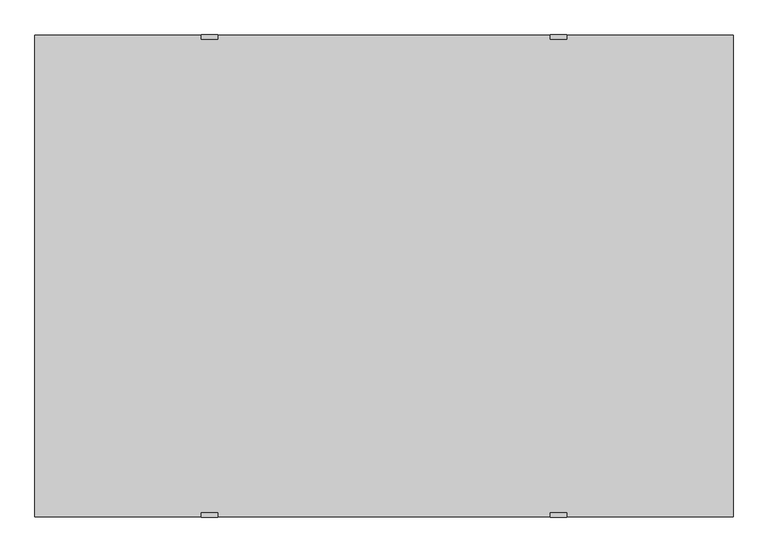
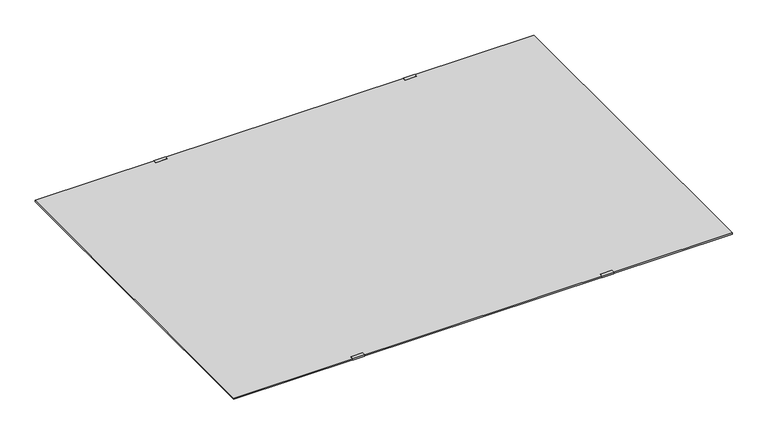
"""IFC4 building model written with IfcOpenShell, lengths in millimetres: proxy geometry."""

from ifc_helpers import new_model, si_unit, frame, origin, origin_with_axes, place, context, project, spatial, polyline, outline, extrude, source, transform, mapped, element, save


def specialty_equipment_58a60da3(model_context):
    return source(origin(), model_context, "Body", "SweptSolid", [
        extrude(outline(polyline([(736.6, 6.35), (723.9, 6.35), (723.9, 7.14375), (737.39375, 7.14375), (737.39375, 0.0), (736.6, 0.0), (736.6, 6.35)])), frame((508.0, 0.0, 0.0), z_axis=(1.0, 0.0, 0.0), x_axis=(0.0, 1.0, 0.0)), (0.0, 0.0, 1.0), 50.8),
        extrude(outline(polyline([(736.6, 6.35), (723.9, 6.35), (723.9, 7.14375), (737.39375, 7.14375), (737.39375, 0.0), (736.6, 0.0), (736.6, 6.35)])), frame((-558.8, 0.0, 0.0), z_axis=(1.0, 0.0, 0.0), x_axis=(0.0, 1.0, 0.0)), (0.0, 0.0, 1.0), 50.8),
        extrude(outline(polyline([(-736.6, 6.35), (-736.6, 0.0), (-737.39375, 0.0), (-737.39375, 7.14375), (-723.9, 7.14375), (-723.9, 6.35), (-736.6, 6.35)])), frame((508.0, 0.0, 0.0), z_axis=(1.0, 0.0, 0.0), x_axis=(0.0, 1.0, 0.0)), (0.0, 0.0, 1.0), 50.8),
        extrude(outline(polyline([(-736.6, 6.35), (-736.6, 0.0), (-737.39375, 0.0), (-737.39375, 7.14375), (-723.9, 7.14375), (-723.9, 6.35), (-736.6, 6.35)])), frame((-558.8, 0.0, 0.0), z_axis=(1.0, 0.0, 0.0), x_axis=(0.0, 1.0, 0.0)), (0.0, 0.0, 1.0), 50.8),
        extrude(outline(polyline([(1066.8, -736.6), (-1066.8, -736.6), (-1066.8, 736.6), (1066.8, 736.6), (1066.8, -736.6)])), origin_with_axes(), (0.0, 0.0, 1.0), 6.35),
    ])


if __name__ == "__main__":
    model = new_model("IFC4")
    model_context = context("Model", 3, world=origin())
    ifc_project = project(units=[si_unit("LENGTHUNIT", "METRE", prefix="MILLI")], contexts=[model_context])
    site = spatial("IfcSite", under=ifc_project)
    building = spatial("IfcBuilding", under=site)
    placement = place(None, origin())
    specialty_equipment_shape = specialty_equipment_58a60da3(model_context)
    element("IfcBuildingElementProxy", 1, Name="Bradley-Washroom_Accessories-Mirrors-747_Standard : 84\" x 36\" + BradEX Womens", ObjectType="Bradley-Washroom_Accessories-Mirrors-747_Standard : 84\" x 36\" + BradEX Womens", at=placement, inside=building, context=model_context, shape_type="MappedRepresentation", body=[
        mapped(specialty_equipment_shape, transform((0.0, 0.0, 0.0), x_axis=(1.0, 0.0, 0.0), y_axis=(0.0, 1.0, 0.0), z_axis=(0.0, 0.0, 1.0))),
    ])
    save(model, "model.ifc")

# Revit data of these elements
# Type "Bradley-Washroom_Accessories-Mirrors-747_Standard : 84\" x 36\" + BradEX Womens"
#   Keynote = "M08831300.01"
#   Warranty Information = "Complete unit, excepting mirrors warranted for one year.\r\n Stainless steel mirror frames for fifteen years.\r\n Plate glass mirrors for fifteen years.\r\n This warranty does not cover installation or any other labor charges and does not apply to any units,\r\n which have been damaged by accident, abuse, improper installation, improper maintenance, or altered in any way."
#   Version = "1.0"
#   URL = "http://www.bradleycorp.com/"
#   Type Comments = "BradEX 1/4\" Float Glass Mirror"
#   OmniClass Title = "Mirrors"
#   OmniClass Code = "23.40.95.17.17"
#   Modeling Code = ""
#   Model = "747-024360"
#   MasterFormat Title = "Commercial Toilet Accessories"
#   MasterFormat Number = "10 28 13. 13"
#   Manufacturer = "Bradley Corporation"
#   Industry Standards = "ASTM C 1036"
#   Fire Rating = "n/a"
#   Description = "Frameless Mirror, Clip Fasteners, 24 by 36 inches"
#   Copyright = "This Model Data is Property of Bradley Corporation"
#   Buy American Act = "Yes"
#   Assembly Code = "C1030900"
#   ADA Compliant = "Yes"
#   Width = 7' - 0"
#   Height = 4' - 10"
#   Fastener Placement = 1' - 9"
#   Depth = 0' - 0 1/4"
#   Default Elevation = 3' - 4"
#   Reflective Material = Glass - Bradley Corp - BradEX - Polished Float Mirror
#   Frame Material = Bradley Corp Stainless Steel - Satin
# Element 1 (IfcBuildingElementProxy, "Bradley-Washroom_Accessories-Mirrors-747_Standard : 84\" x 36\" + BradEX Womens")
#   Materials on its faces: "Bradley Corp Stainless Steel - Satin", "Glass - Bradley Corp - BradEX - Polished Float Mirror"
# Materials
#   "Glass - Bradley Corp - BradEX - Polished Float Mirror": class "Glass", colour RGB 221 230 232, transparency 0, Manufacturer = "Bradley Corporation", URL = "www.bradleycorp.com", Description = "Stainless Steel - Satin Finish", Cost = 0
#   "Bradley Corp Stainless Steel - Satin": class "Metal", colour RGB 189 187 185, transparency 0, Manufacturer = "Bradley Corporation", URL = "www.bradleycorp.com", Description = "Stainless Steel - Satin Finish", Cost = 0
